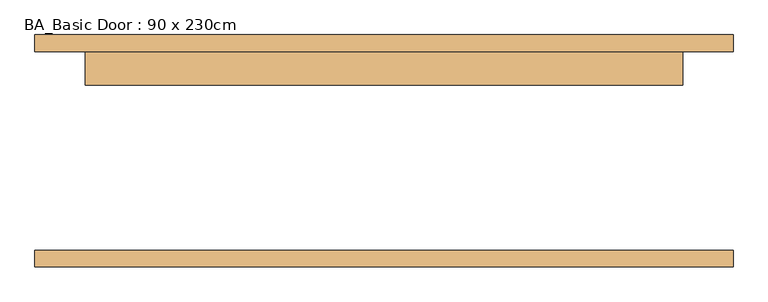
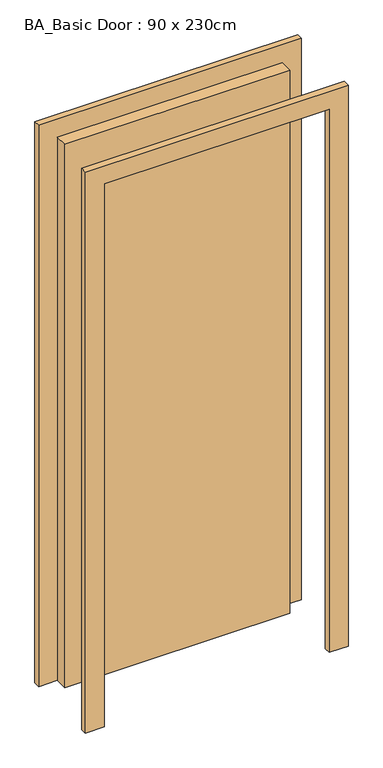
"""IFC4 building model written with IfcOpenShell, lengths in millimetres: door geometry, BA_Basic Door : 90 x 230cm."""

from ifc_helpers import new_model, si_unit, frame, origin, origin_with_axes, place, context, project, spatial, polyline, outline, extrude, source, transform, mapped, element, save


def ba_basic_door_90_x_230cm_e5931120(model_context):
    return source(origin(), model_context, "Body", "SweptSolid", [
        extrude(outline(polyline([(450.0, 99.0), (-450.0, 99.0), (-450.0, 150.0), (450.0, 150.0), (450.0, 99.0)])), origin_with_axes(), (0.0, 0.0, 1.0), 2300.0),
        extrude(outline(polyline([(2376.0, -526.0), (0.0, -526.0), (0.0, -450.0), (2300.0, -450.0), (2300.0, 450.0), (0.0, 450.0), (0.0, 526.0), (2376.0, 526.0), (2376.0, -526.0)])), frame((0.0, 150.0, 0.0), z_axis=(0.0, 1.0, 0.0), x_axis=(0.0, 0.0, 1.0)), (0.0, 0.0, 1.0), 25.0),
        extrude(outline(polyline([(2376.0, 526.0), (2376.0, -526.0), (0.0, -526.0), (0.0, -450.0), (2300.0, -450.0), (2300.0, 450.0), (0.0, 450.0), (0.0, 526.0), (2376.0, 526.0)])), frame((0.0, -175.0, 0.0), z_axis=(0.0, 1.0, 0.0), x_axis=(0.0, 0.0, 1.0)), (0.0, 0.0, 1.0), 25.0),
    ])


if __name__ == "__main__":
    model = new_model("IFC4")
    model_context = context("Model", 3, world=origin())
    ifc_project = project(units=[si_unit("LENGTHUNIT", "METRE", prefix="MILLI")], contexts=[model_context])
    site = spatial("IfcSite", under=ifc_project)
    building = spatial("IfcBuilding", under=site)
    placement = place(None, origin())
    ba_basic_door_90_x_230cm_shape = ba_basic_door_90_x_230cm_e5931120(model_context)
    element("IfcDoor", 1, ObjectType="BA_Basic Door : 90 x 230cm", at=placement, inside=building, context=model_context, shape_type="MappedRepresentation", body=[
        mapped(ba_basic_door_90_x_230cm_shape, transform((0.0, 0.0, 0.0), x_axis=(1.0, 0.0, 0.0), y_axis=(0.0, 1.0, 0.0), z_axis=(0.0, 0.0, 1.0))),
    ])
    save(model, "model.ifc")

# Revit data of these elements
# Type "BA_Basic Door : 90 x 230cm"
#   Type Mark = "43"
#   Construction Type Id = "MDOOR"
#   Analytic Construction = "Metal"
#   Window height [instance default] = 1000 mm
#   Thickness = 51 mm
#   Thermal Resistance (R) = 0.270117 (m²·K)/W
#   Cut [instance default] = -100 mm
#   Heat Transfer Coefficient (U) = 3.7021 W/(m²·K)
#   Height = 2300 mm
#   Trim Projection Ext = 25 mm
#   Trim Projection Int = 25 mm
#   Trim Width = 76 mm
#   Width = 900 mm
#   Door window [instance default] = no
#   Define Thermal Properties by = 1
#   Door Material = Default
#   Frame Material = Default
#   Visual Light Transmittance = 0
#   Solar Heat Gain Coefficient = 0
#   Function = (empty or 0)
#   Wall Closure = (empty or 0)
# Element 1 (IfcDoor, "BA_Basic Door : 90 x 230cm")
#   Materials on its faces: "Default"
# Materials
#   "Default": class "Generic", colour RGB 255 255 255, transparency 0, Cost = 0
